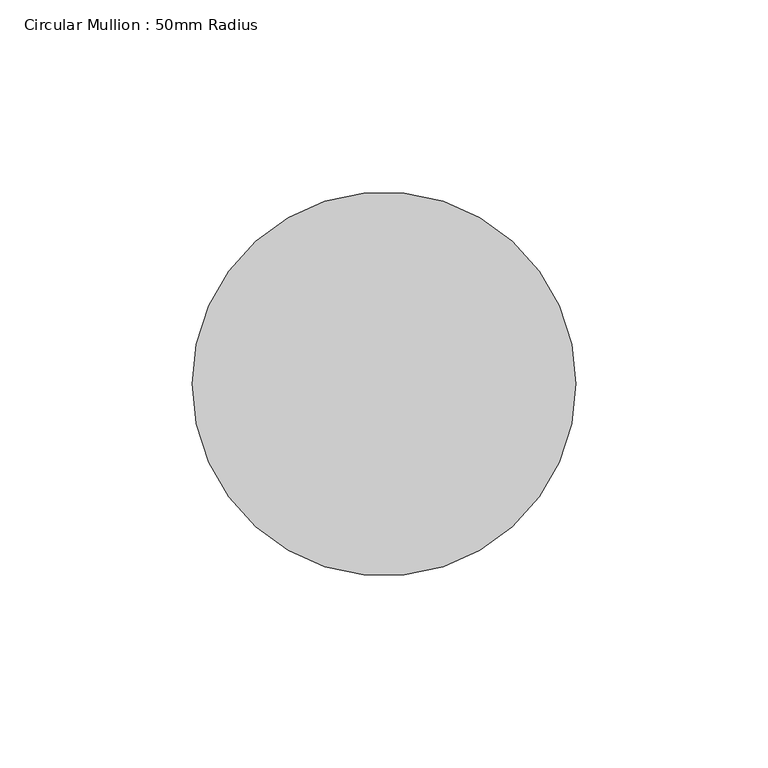
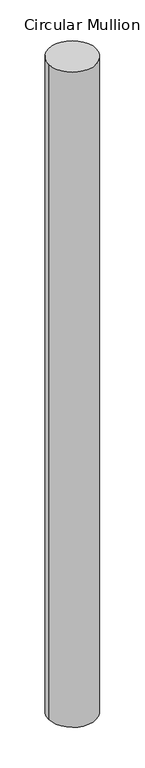
"""IFC4 building model written with IfcOpenShell, lengths in millimetres: member geometry, Circular Mullion : 50mm Radius."""

from ifc_helpers import new_model, si_unit, frame, origin, place, context, project, spatial, circle_curve, ellipse_curve, source, transform, mapped, element, save
from ifc_brep_helpers import plane_surface, cylinder_surface, advanced_brep


def circular_mullion_50mm_radius_6e0bbbb8(model_context):
    return source(origin(), model_context, "Body", "AdvancedBrep", [
        advanced_brep(
        [(0.0, 0.0, 0.0), (-100.0, 0.0, 0.0), (0.0, 0.0, -1449.8327894), (-100.0, 0.0, -1450.2200218)],
        [
            (0, 1, circle_curve(frame((-50.0, 0.0, 0.0), z_axis=(0.0, 0.0, 1.0), x_axis=(1.0, 0.0, 0.0)), 50.0)),
            (1, 0, circle_curve(frame((-50.0, 0.0, 0.0), z_axis=(0.0, 0.0, 1.0), x_axis=(1.0, 0.0, 0.0)), 50.0)),
            (0, 2),
            (2, 3, ellipse_curve(frame((-50.0, 0.0, -1450.0264056), z_axis=(-0.003871909342754237, -0.014106902170600248, 0.9998929960896769), x_axis=(0.26465219623786995, 0.9642329690773194, 0.014628614794623313)), 50.0053508, 50.0)),
            (3, 1),
            (3, 2, ellipse_curve(frame((-50.0, 0.0, -1450.0264056), z_axis=(-0.003871909342754237, -0.014106902170600248, 0.9998929960896769), x_axis=(0.26465219623786995, 0.9642329690773194, 0.014628614794623313)), 50.0053508, 50.0)),
        ],
        [
            plane_surface(frame((0.0, -100.0, 0.0), z_axis=(0.0, 0.0, 1.0), x_axis=(-1.0, 0.0, 0.0))),
            cylinder_surface(frame((-50.0, 0.0, 0.0), z_axis=(0.0, 0.0, 1.0), x_axis=(1.0, 0.0, 0.0)), 50.0),
            plane_surface(frame((-293.9296606, 80.6746219, -1449.8327894), z_axis=(0.003871909342754238, 0.014106902170600252, -0.9998929960896771), x_axis=(0.2646521962378699, 0.9642329690773194, 0.014628614794620631))),
        ],
        [
            (0, [[1, 2]]),
            (1, [[-1, 3, 4, 5]]),
            (1, [[-2, -5, 6, -3]]),
            (2, [[-6, -4]]),
        ],
    ),
    ])


if __name__ == "__main__":
    model = new_model("IFC4")
    model_context = context("Model", 3, world=origin())
    ifc_project = project(units=[si_unit("LENGTHUNIT", "METRE", prefix="MILLI")], contexts=[model_context])
    site = spatial("IfcSite", under=ifc_project)
    building = spatial("IfcBuilding", under=site)
    placement = place(None, origin())
    circular_mullion_50mm_radius_shape = circular_mullion_50mm_radius_6e0bbbb8(model_context)
    element("IfcMember", 1, ObjectType="Circular Mullion : 50mm Radius", at=placement, inside=building, context=model_context, shape_type="MappedRepresentation", body=[
        mapped(circular_mullion_50mm_radius_shape, transform((0.0, 0.0, 0.0), x_axis=(1.0, 0.0, 0.0), y_axis=(0.0, 1.0, 0.0), z_axis=(0.0, 0.0, 1.0))),
    ])
    save(model, "model.ifc")

# Revit data of these elements
# Type "Circular Mullion : 50mm Radius"
#   built-in parameter 1007350 = 0.164042 (stored number, unit not read)
# Element 1 (IfcMember, "Circular Mullion : 50mm Radius")
#   Materials on its faces: "Aluminium"
# Materials
#   "Aluminium": class "Metal", colour RGB 247 247 247, transparency 0, Description = "Aluminium 6061", Cost = 0
